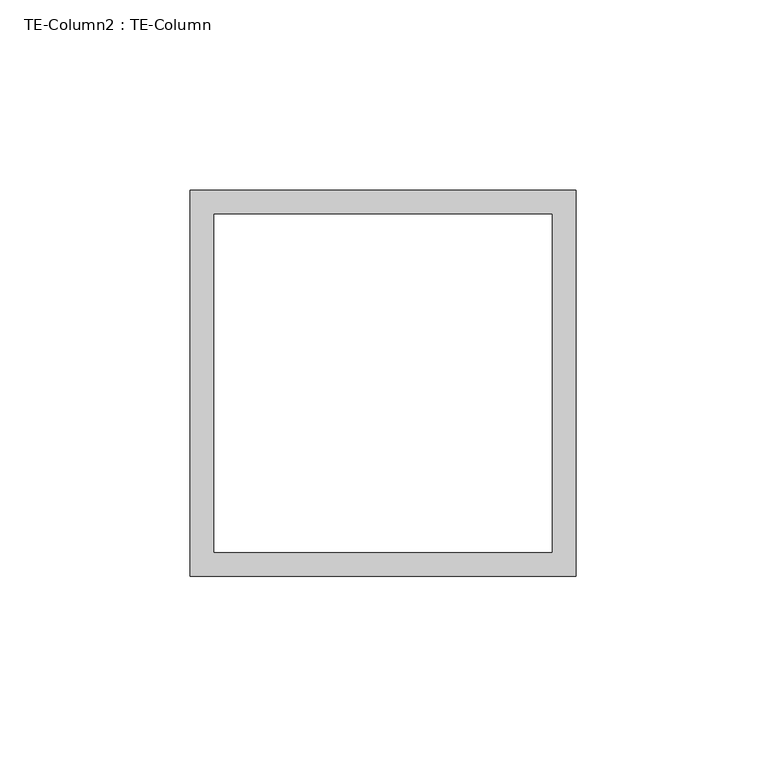
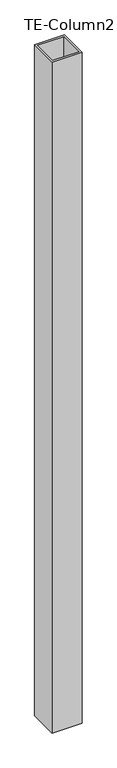
"""IFC4 building model written with IfcOpenShell, lengths in millimetres: proxy geometry, TE-Column2 : TE-Column."""

import ifcopenshell
import ifcopenshell.guid

model = None  # the IFC model being written
_history = None  # IfcOwnerHistory: only IFC2X3 demands one
_inside = {}  # id of a spatial element -> (the spatial element, [elements in it])
_under = {}  # id of a project, library or spatial element -> (it, [spatial elements below it])
_declared = {}  # id of a project -> (the project, [libraries it declares])
_typed = {}  # id of a type object -> (the type object, [elements of that type])
_made_of = {}  # id of a material, layer set ... -> (it, [elements and type objects made of it])


def new_model(schema):
    """Start an empty IFC model of exactly this schema.

    Asked for "IFC4X3", IfcOpenShell would pick the latest addendum, in which some entities
    have other attributes; the version numbers below select the first issue.
    IFC2X3 requires an IfcOwnerHistory on every rooted entity: one is made here for all.
    """
    global model, _history
    if schema == "IFC4X3":
        model = ifcopenshell.file(schema_version=(4, 3, 0, 0))
    else:
        model = ifcopenshell.file(schema=schema)
    _inside.clear()
    _under.clear()
    _declared.clear()
    _typed.clear()
    _made_of.clear()
    _history = None
    if model.schema == "IFC2X3":
        org = make("IfcOrganization", Name="unknown")
        user = make(
            "IfcPersonAndOrganization",
            ThePerson=make("IfcPerson", FamilyName="unknown"),
            TheOrganization=org,
        )
        app = make(
            "IfcApplication",
            ApplicationDeveloper=org,
            Version="unknown",
            ApplicationFullName="unknown",
            ApplicationIdentifier="unknown",
        )
        _history = make(
            "IfcOwnerHistory",
            OwningUser=user,
            OwningApplication=app,
            ChangeAction="ADDED",
            CreationDate=0,
        )
    return model


def make(cls, **values):
    """One entity of the class cls with the attributes given. An attribute that is None is left unset."""
    return model.create_entity(
        cls, **{name: value for name, value in values.items() if value is not None}
    )


def rooted(cls, **values):
    """An entity with a GlobalId (a new one), such as an element, a storey or a relation."""
    return make(cls, GlobalId=ifcopenshell.guid.new(), OwnerHistory=_history, **values)


def si_unit(unit_type, name, prefix=None):
    """IfcSIUnit, for example si_unit("LENGTHUNIT", "METRE", prefix="MILLI")."""
    return make("IfcSIUnit", UnitType=unit_type, Prefix=prefix, Name=name)


def assignment(units):
    """IfcUnitAssignment: the units of a project."""
    return None if units is None else make("IfcUnitAssignment", Units=units)


def point(xyz):
    """IfcCartesianPoint."""
    return None if xyz is None else make("IfcCartesianPoint", Coordinates=xyz)


def direction(xyz):
    """IfcDirection."""
    return None if xyz is None else make("IfcDirection", DirectionRatios=xyz)


def frame(location, z_axis=None, x_axis=None):
    """IfcAxis2Placement3D, a coordinate frame: its origin and axes. An axis left out is left unset."""
    return make(
        "IfcAxis2Placement3D",
        Location=point(location),
        Axis=direction(z_axis),
        RefDirection=direction(x_axis),
    )


def origin():
    """The frame at (0, 0, 0) with its axes left unset."""
    return frame((0.0, 0.0, 0.0))


def place(relative_to, where):
    """IfcLocalPlacement: puts the frame where relative to a parent placement (None: the world)."""
    return make(
        "IfcLocalPlacement", PlacementRelTo=relative_to, RelativePlacement=where
    )


def context(
    kind, dimensions, precision=None, world=None, true_north=None, identifier=None
):
    """IfcGeometricRepresentationContext, for example the 3D "Model" context."""
    return make(
        "IfcGeometricRepresentationContext",
        ContextIdentifier=identifier,
        ContextType=kind,
        CoordinateSpaceDimension=dimensions,
        Precision=precision,
        WorldCoordinateSystem=world,
        TrueNorth=true_north,
    )


def project(units=None, contexts=None):
    """IfcProject with its units and contexts."""
    return rooted(
        "IfcProject",
        Name="project",
        RepresentationContexts=contexts,
        UnitsInContext=assignment(units),
    )


def spatial(cls, under=None, at=None, **own):
    """A site, building, storey or space (cls), placed at a placement, below another one or the project."""
    s = rooted(cls, ObjectPlacement=at, **own)
    if under is not None:
        _under.setdefault(under.id(), (under, []))[1].append(s)
    return s


def polyline(points):
    """IfcPolyline through the points."""
    return make("IfcPolyline", Points=[point(p) for p in points])


def outline(outer, holes=None, kind="AREA"):
    """IfcArbitraryClosedProfileDef: a profile drawn as a closed curve; with holes, ...WithVoids."""
    if holes is None:
        return make("IfcArbitraryClosedProfileDef", ProfileType=kind, OuterCurve=outer)
    return make(
        "IfcArbitraryProfileDefWithVoids",
        ProfileType=kind,
        OuterCurve=outer,
        InnerCurves=holes,
    )


def extrude(swept, where, along, depth):
    """IfcExtrudedAreaSolid: the profile swept, set in the frame where, extruded along a direction by depth."""
    return make(
        "IfcExtrudedAreaSolid",
        SweptArea=swept,
        Position=where,
        ExtrudedDirection=direction(along),
        Depth=depth,
    )


def shape(context_of_items, identifier, shape_type, items):
    """IfcShapeRepresentation: the items that make up one representation, for example the "Body"."""
    return make(
        "IfcShapeRepresentation",
        ContextOfItems=context_of_items,
        RepresentationIdentifier=identifier,
        RepresentationType=shape_type,
        Items=items,
    )


def source(mapping_origin, context_of_items, identifier, shape_type, items):
    """IfcRepresentationMap: a shape defined once, which mapped items show again and again."""
    return make(
        "IfcRepresentationMap",
        MappingOrigin=mapping_origin,
        MappedRepresentation=shape(context_of_items, identifier, shape_type, items),
    )


def transform(
    local_origin,
    x_axis=None,
    y_axis=None,
    z_axis=None,
    scale=None,
    scale2=None,
    scale3=None,
    uniform=True,
):
    """IfcCartesianTransformationOperator3D, or its non-uniform kind. x_axis, y_axis, z_axis: its Axis1, 2, 3."""
    if uniform:
        return make(
            "IfcCartesianTransformationOperator3D",
            Axis1=direction(x_axis),
            Axis2=direction(y_axis),
            LocalOrigin=point(local_origin),
            Scale=scale,
            Axis3=direction(z_axis),
        )
    return make(
        "IfcCartesianTransformationOperator3DnonUniform",
        Axis1=direction(x_axis),
        Axis2=direction(y_axis),
        LocalOrigin=point(local_origin),
        Scale=scale,
        Axis3=direction(z_axis),
        Scale2=scale2,
        Scale3=scale3,
    )


def mapped(mapping_source, mapping_target):
    """IfcMappedItem: shows the shape of a source again, moved by a transform."""
    return make(
        "IfcMappedItem", MappingSource=mapping_source, MappingTarget=mapping_target
    )


def made_of(thing, what):
    """Note that an element or type object is made of a material, layer set ...; save() writes the relation."""
    if what is not None:
        _made_of.setdefault(what.id(), (what, []))[1].append(thing)
    return thing


def element(
    cls,
    number,
    at=None,
    inside=None,
    cuts=None,
    type_object=None,
    material=None,
    context=None,
    identifier="Body",
    shape_type=None,
    held_by="IfcProductDefinitionShape",
    body=None,
    shapes=None,
    **own,
):
    """One element of the class cls, such as IfcWall. Its Tag is "e" and its number.

    at: its placement. inside: the storey or other place that contains it. cuts: it is an
    opening in that element (IfcRelVoidsElement). A single representation is given by context,
    identifier, shape_type and body (its items); several are given by shapes. held_by: the class
    of the entity that holds the representations. save() writes the other relations.
    """
    e = rooted(cls, Tag="e%d" % number, ObjectPlacement=at, **own)
    if body is not None:
        shapes = [shape(context, identifier, shape_type, body)]
    if shapes is not None:
        e.Representation = make(held_by, Representations=shapes)
    if inside is not None:
        _inside.setdefault(inside.id(), (inside, []))[1].append(e)
    if cuts is not None:
        rooted(
            "IfcRelVoidsElement", RelatingBuildingElement=cuts, RelatedOpeningElement=e
        )
    if type_object is not None:
        _typed.setdefault(type_object.id(), (type_object, []))[1].append(e)
    return made_of(e, material)


def aggregate(whole, parts):
    """IfcRelAggregates: a whole, such as a stair, and the parts it consists of."""
    return rooted("IfcRelAggregates", RelatingObject=whole, RelatedObjects=parts)


def save(model, path):
    """Write the relations noted so far, then the file.

    IfcRelAggregates (storeys below a building ...), IfcRelContainedInSpatialStructure (elements
    in a storey), IfcRelDefinesByType, IfcRelAssociatesMaterial and IfcRelDeclares: one each for
    every whole, place, type object, material and project.
    """
    for whole, parts in _under.values():
        aggregate(whole, parts)
    for where, things in _inside.values():
        rooted(
            "IfcRelContainedInSpatialStructure",
            RelatedElements=things,
            RelatingStructure=where,
        )
    for kind, things in _typed.values():
        rooted("IfcRelDefinesByType", RelatedObjects=things, RelatingType=kind)
    for what, things in _made_of.values():
        rooted("IfcRelAssociatesMaterial", RelatedObjects=things, RelatingMaterial=what)
    for by, libraries in _declared.values():
        rooted("IfcRelDeclares", RelatingContext=by, RelatedDefinitions=libraries)
    model.write(path)


def te_column2_te_column_b03e1283(model_context):
    return source(origin(), model_context, "Body", "SweptSolid", [
        extrude(outline(polyline([(590318.6434739, -531667.7913841), (590318.6434739, -531769.3913841), (590217.0434739, -531769.3913841), (590217.0434739, -531667.7913841), (590318.6434739, -531667.7913841)]), holes=[polyline([(590223.3934739, -531674.1413841), (590223.3934739, -531763.0413841), (590312.2934739, -531763.0413841), (590312.2934739, -531674.1413841), (590223.3934739, -531674.1413841)])]), frame((0.0, 0.0, 28.575), z_axis=(0.0, 0.0, 1.0), x_axis=(1.0, 0.0, 0.0)), (0.0, 0.0, 1.0), 2406.65),
    ])


if __name__ == "__main__":
    model = new_model("IFC4")
    model_context = context("Model", 3, world=origin())
    ifc_project = project(units=[si_unit("LENGTHUNIT", "METRE", prefix="MILLI")], contexts=[model_context])
    site = spatial("IfcSite", under=ifc_project)
    building = spatial("IfcBuilding", under=site)
    placement = place(None, origin())
    te_column2_te_column_shape = te_column2_te_column_b03e1283(model_context)
    element("IfcBuildingElementProxy", 1, Name="TE-Column2 : TE-Column", ObjectType="TE-Column2 : TE-Column", at=placement, inside=building, context=model_context, shape_type="MappedRepresentation", body=[
        mapped(te_column2_te_column_shape, transform((0.0, 0.0, 0.0), x_axis=(1.0, 0.0, 0.0), y_axis=(0.0, 1.0, 0.0), z_axis=(0.0, 0.0, 1.0))),
    ])
    save(model, "model.ifc")

# Revit data of these elements
# Element 1 (IfcBuildingElementProxy, "TE-Column2 : TE-Column")
#   Materials on its faces: "4\"X4\" GALV. HSS TUBING"
# Materials
#   "4\"X4\" GALV. HSS TUBING": class "Generic", colour RGB 211 211 207, transparency 0, Cost = 0
